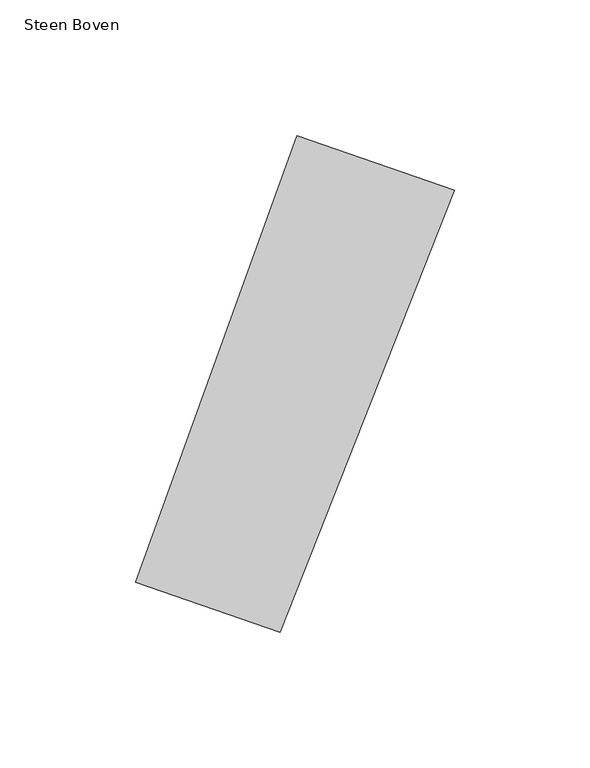
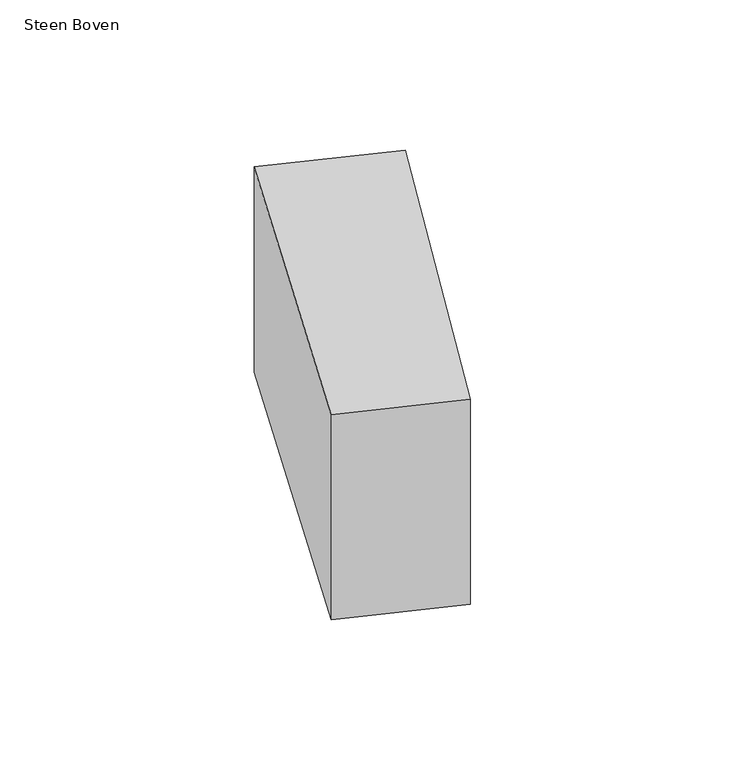
"""IFC4 building model written with IfcOpenShell, lengths in millimetres: proxy geometry, 00_GMA_steen_versie_4 : Steen Boven."""

from ifc_helpers import new_model, si_unit, origin, origin_with_axes, place, context, project, spatial, polyline, outline, extrude, source, transform, mapped, element, save


def steen_boven_7bdc508c(model_context):
    return source(origin(), model_context, "Body", "SweptSolid", [
        extrude(outline(polyline([(133.8476162, 154.0405972), (69.6391787, -8.9318763), (16.3021415, 9.4888401), (75.7830876, 174.0900339), (133.8476162, 154.0405972)])), origin_with_axes(), (0.0, 0.0, 1.0), 100.0),
    ])


if __name__ == "__main__":
    model = new_model("IFC4")
    model_context = context("Model", 3, world=origin())
    ifc_project = project(units=[si_unit("LENGTHUNIT", "METRE", prefix="MILLI")], contexts=[model_context])
    site = spatial("IfcSite", under=ifc_project)
    building = spatial("IfcBuilding", under=site)
    placement = place(None, origin())
    steen_boven_shape = steen_boven_7bdc508c(model_context)
    element("IfcBuildingElementProxy", 1, Name="00_GMA_steen_versie_4 : Steen Boven", ObjectType="00_GMA_steen_versie_4 : Steen Boven", at=placement, inside=building, context=model_context, shape_type="MappedRepresentation", body=[
        mapped(steen_boven_shape, transform((0.0, 0.0, 0.0), x_axis=(1.0, 0.0, 0.0), y_axis=(0.0, 1.0, 0.0), z_axis=(0.0, 0.0, 1.0))),
    ])
    save(model, "model.ifc")

# Revit data of these elements
# Type "00_GMA_steen_versie_4 : Steen Boven"
#   StootVoegHalfBoven [instance default] = 5 mm
#   StootVoegHalf [instance default] = 5 mm
#   StootVoegBreedteOnder = 10 mm
#   StootVoegBreedteBoven = 10 mm
#   Steendikte = 100 mm
#   LintVoegOnderHalf = 5 mm
#   LintVoegOnder = 10 mm
#   LintVoegBovenHalf = 0 mm
#   LintVoegBoven = 0 mm
#   materiaal = none
#   MateriaalVoeg = none
#   Default Elevation = 0
